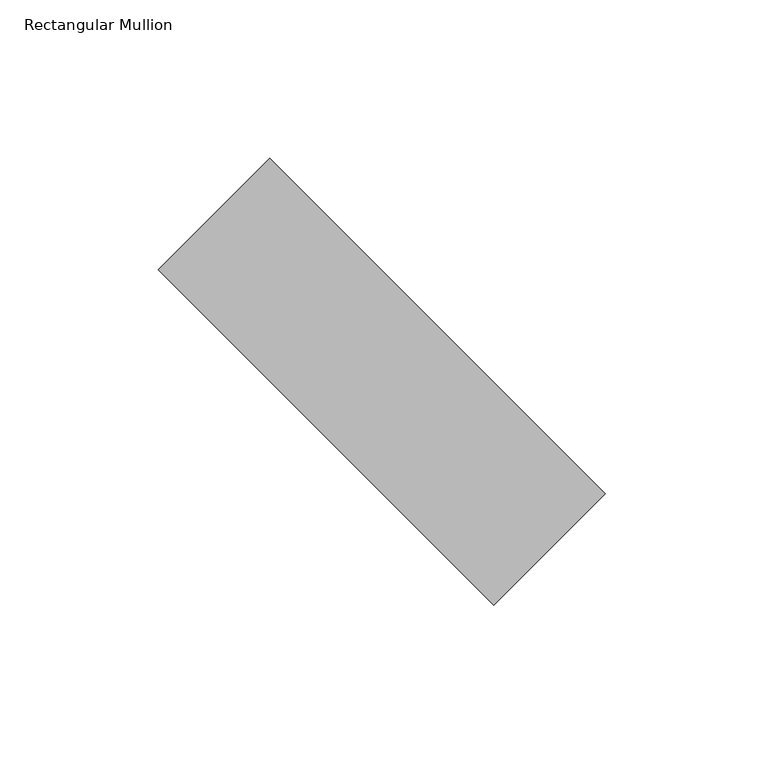
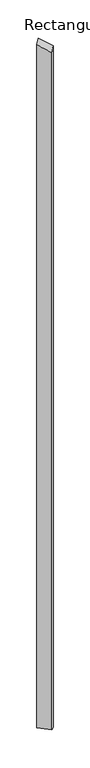
"""IFC4 building model written with IfcOpenShell, lengths in millimetres: member geometry, Rectangular Mullion : tilted mullions."""

from ifc_helpers import new_model, si_unit, origin, place, context, project, spatial, faceted_brep, source, transform, mapped, element, save


def rectangular_mullion_a716d863(model_context):
    return source(origin(), model_context, "Body", "Brep", [
        faceted_brep([(-35.3553391, 70.7106781, -7999.6208242), (70.7106781, -35.3553391, -7999.6208242), (35.3553391, -70.7106781, -7999.6208242), (-70.7106781, 35.3553391, -7999.6208242), (-70.7106781, 35.3553391, 10.1931486), (-35.3553391, 70.7106781, 55.1927576), (35.3553391, -70.7106781, -55.1927576), (70.7106781, -35.3553391, -10.1931486)], [[[0, 1, 2, 3]], [[4, 5, 0, 3]], [[6, 4, 3, 2]], [[7, 6, 2, 1]], [[5, 7, 1, 0]], [[5, 4, 6, 7]]]),
    ])


if __name__ == "__main__":
    model = new_model("IFC4")
    model_context = context("Model", 3, world=origin())
    ifc_project = project(units=[si_unit("LENGTHUNIT", "METRE", prefix="MILLI")], contexts=[model_context])
    site = spatial("IfcSite", under=ifc_project)
    building = spatial("IfcBuilding", under=site)
    placement = place(None, origin())
    rectangular_mullion_shape = rectangular_mullion_a716d863(model_context)
    element("IfcMember", 1, ObjectType="Rectangular Mullion : tilted mullions", at=placement, inside=building, context=model_context, shape_type="MappedRepresentation", body=[
        mapped(rectangular_mullion_shape, transform((0.0, 0.0, 0.0), x_axis=(1.0, 0.0, 0.0), y_axis=(0.0, 1.0, 0.0), z_axis=(0.0, 0.0, 1.0))),
    ])
    save(model, "model.ifc")

# Revit data of these elements
# Type "Rectangular Mullion : tilted mullions"
#   built-in parameter 1007304 = 0.492126 (stored number, unit not read)
#   built-in parameter 1007301 = 0.082021 (stored number, unit not read)
#   built-in parameter 1007300 = 0.082021 (stored number, unit not read)
# Element 1 (IfcMember, "Rectangular Mullion : tilted mullions")
#   Materials on its faces: "Aluminum"
# Materials
#   "Aluminum": class "Metal", colour RGB 244 244 244, transparency 0, Description = "Aluminum 6061", Cost = 0
